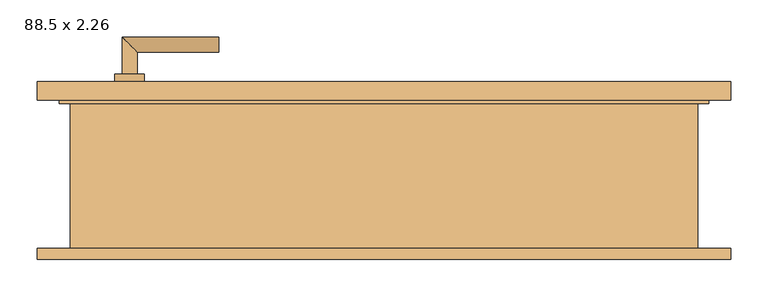
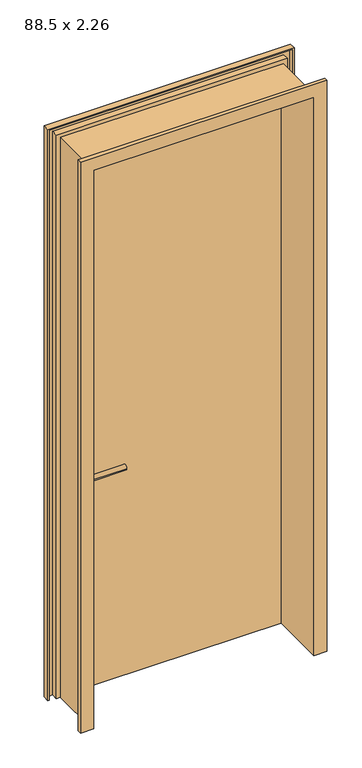
"""IFC4 building model written with IfcOpenShell, lengths in millimetres: door geometry, Drehflügel 1-flg - Stahlzarge : 88.5 x 2.26."""

from ifc_helpers import new_model, si_unit, point, frame, frame_2d, origin, origin_with_axes, place, context, project, spatial, polyline, circle_curve, ellipse_curve, trimmed, segment, composite_curve, outline, extrude, faceted_brep, source, transform, mapped, element, save
from ifc_brep_helpers import plane_surface, cylinder_surface, advanced_brep


def door_88_5_x_2_26_7d47f87c(model_context):
    return source(origin(), model_context, "Body", "SolidModel", [
        advanced_brep(
        [(-352.5, 89.4346141, 900.0), (-332.5, 89.4346141, 900.0), (-352.5, 19.4346141, 900.0), (-332.5, 39.4346141, 900.0), (-222.5, 19.4346141, 900.0), (-222.5, 39.4346141, 900.0)],
        [
            (0, 1, circle_curve(frame((-342.5, 89.4346141, 900.0), z_axis=(0.0, 1.0, 0.0), x_axis=(1.0, 0.0, 0.0)), 10.0)),
            (1, 0, circle_curve(frame((-342.5, 89.4346141, 900.0), z_axis=(0.0, 1.0, 0.0), x_axis=(1.0, 0.0, 0.0)), 10.0)),
            (0, 2),
            (2, 3, ellipse_curve(frame((-342.5, 29.4346141, 900.0), z_axis=(-0.7071067811865385, 0.7071067811865565, 0.0), x_axis=(0.7071067811865563, 0.7071067811865386, 0.0)), 14.1421356, 10.0)),
            (3, 1),
            (3, 2, ellipse_curve(frame((-342.5, 29.4346141, 900.0), z_axis=(-0.7071067811865385, 0.7071067811865565, 0.0), x_axis=(0.7071067811865563, 0.7071067811865386, 0.0)), 14.1421356, 10.0)),
            (4, 5, circle_curve(frame((-222.5, 29.4346141, 900.0), z_axis=(1.0, 0.0, 0.0), x_axis=(0.0, 1.0, 0.0)), 10.0)),
            (5, 4, circle_curve(frame((-222.5, 29.4346141, 900.0), z_axis=(1.0, 0.0, 0.0), x_axis=(0.0, 1.0, 0.0)), 10.0)),
            (2, 4),
            (5, 3),
        ],
        [
            plane_surface(frame((-342.5, 89.4346141, -387.7526403), z_axis=(0.0, 1.0, 0.0), x_axis=(0.0, 0.0, 1.0))),
            cylinder_surface(frame((-342.5, 89.4346141, 900.0), z_axis=(0.0, 1.0, 0.0), x_axis=(1.0, 0.0, 0.0)), 10.0),
            plane_surface(frame((-222.5, 29.4346141, -387.7526403), z_axis=(1.0, 0.0, 0.0), x_axis=(0.0, 0.0, 1.0))),
            cylinder_surface(frame((-342.5, 29.4346141, 900.0), z_axis=(-1.0, 0.0, 0.0), x_axis=(0.0, 1.0, 0.0)), 10.0),
        ],
        [
            (0, [[1, 2]]),
            (1, [[-1, 3, 4, 5]]),
            (1, [[-2, -5, 6, -3]]),
            (2, [[7, 8]]),
            (3, [[-4, 9, -8, 10]]),
            (3, [[-6, -10, -7, -9]]),
        ],
    ),
        advanced_brep(
        [(-332.5, 149.4346141, 900.0), (-352.5, 149.4346141, 900.0), (-332.5, 179.4346141, 900.0), (-352.5, 199.4346141, 900.0), (-222.5, 179.4346141, 900.0), (-222.5, 199.4346141, 900.0)],
        [
            (0, 1, circle_curve(frame((-342.5, 149.4346141, 900.0), z_axis=(0.0, -1.0, 0.0), x_axis=(-1.0, 0.0, 0.0)), 10.0)),
            (1, 0, circle_curve(frame((-342.5, 149.4346141, 900.0), z_axis=(0.0, -1.0, 0.0), x_axis=(-1.0, 0.0, 0.0)), 10.0)),
            (0, 2),
            (2, 3, ellipse_curve(frame((-342.5, 189.4346141, 900.0), z_axis=(-0.7071067811865475, -0.7071067811865475, 0.0), x_axis=(0.7071067811865474, -0.7071067811865476, 0.0)), 14.1421356, 10.0)),
            (3, 1),
            (3, 2, ellipse_curve(frame((-342.5, 189.4346141, 900.0), z_axis=(-0.7071067811865475, -0.7071067811865475, 0.0), x_axis=(0.7071067811865474, -0.7071067811865476, 0.0)), 14.1421356, 10.0)),
            (4, 5, circle_curve(frame((-222.5, 189.4346141, 900.0), z_axis=(1.0, 0.0, 0.0), x_axis=(0.0, 1.0, 0.0)), 10.0)),
            (5, 4, circle_curve(frame((-222.5, 189.4346141, 900.0), z_axis=(1.0, 0.0, 0.0), x_axis=(0.0, 1.0, 0.0)), 10.0)),
            (2, 4),
            (5, 3),
        ],
        [
            plane_surface(frame((-342.5, 149.4346141, -387.7526403), z_axis=(0.0, -1.0, 0.0), x_axis=(0.0, 0.0, 1.0))),
            cylinder_surface(frame((-342.5, 149.4346141, 900.0), z_axis=(0.0, -1.0, 0.0), x_axis=(-1.0, 0.0, 0.0)), 10.0),
            plane_surface(frame((-222.5, 189.4346141, -387.7526403), z_axis=(1.0, 0.0, 0.0), x_axis=(0.0, 0.0, 1.0))),
            cylinder_surface(frame((-342.5, 189.4346141, 900.0), z_axis=(-1.0, 0.0, 0.0), x_axis=(0.0, 1.0, 0.0)), 10.0),
        ],
        [
            (0, [[1, 2]]),
            (1, [[-1, 3, 4, 5]]),
            (1, [[-2, -5, 6, -3]]),
            (2, [[7, 8]]),
            (3, [[-4, 9, -8, 10]]),
            (3, [[-6, -10, -7, -9]]),
        ],
    ),
        extrude(outline(composite_curve([segment(trimmed(circle_curve(frame_2d((900.0, -342.5)), 20.0), [point((900.0, -362.5))], [point((900.0, -322.5))], False, "CARTESIAN"), True, "CONTINUOUS"), segment(trimmed(circle_curve(frame_2d((900.0, -342.5)), 20.0), [point((900.0, -322.5))], [point((900.0, -362.5))], False, "CARTESIAN"), True, "CONTINUOUS")], self_intersect=False)), frame((0.0, 79.4346141, 0.0), z_axis=(0.0, 1.0, 0.0), x_axis=(0.0, 0.0, 1.0)), (0.0, 0.0, 1.0), 10.0),
        extrude(outline(composite_curve([segment(trimmed(circle_curve(frame_2d((900.0, -342.5)), 20.0), [point((900.0, -362.5))], [point((900.0, -322.5))], False, "CARTESIAN"), True, "CONTINUOUS"), segment(trimmed(circle_curve(frame_2d((900.0, -342.5)), 20.0), [point((900.0, -322.5))], [point((900.0, -362.5))], False, "CARTESIAN"), True, "CONTINUOUS")], self_intersect=False)), frame((0.0, 139.4346141, 0.0), z_axis=(0.0, 1.0, 0.0), x_axis=(0.0, 0.0, 1.0)), (0.0, 0.0, 1.0), 10.0),
        extrude(outline(polyline([(432.5, 114.4346141), (-432.5, 114.4346141), (-432.5, 139.4346141), (432.5, 139.4346141), (432.5, 114.4346141)])), origin_with_axes(), (0.0, 0.0, 1.0), 2250.0),
        faceted_brep([(466.9603207, -100.5653859, 0.0), (417.5, -100.5653859, 0.0), (417.5, 114.4346141, 0.0), (432.5, 114.4346141, 0.0), (432.5, 139.4346141, 0.0), (466.9603207, 139.4346141, 0.0), (466.9603207, 114.4346141, 0.0), (461.9603207, 114.4346141, 0.0), (461.9603207, 134.4346141, 0.0), (437.5, 134.4346141, 0.0), (437.5, 109.4346141, 0.0), (422.5, 109.4346141, 0.0), (422.5, -95.5653859, 0.0), (461.9603207, -95.5653859, 0.0), (461.9603207, -85.5653859, 0.0), (466.9603207, -85.5653859, 0.0), (466.9603207, -100.5653859, 2284.4603207), (-466.9603207, -100.5653859, 2284.4603207), (-466.9603207, -100.5653859, 0.0), (-417.5, -100.5653859, 0.0), (-417.5, -100.5653859, 2235.0), (417.5, -100.5653859, 2235.0), (417.5, 114.4346141, 2235.0), (-417.5, 114.4346141, 2235.0), (-417.5, 114.4346141, 0.0), (-432.5, 114.4346141, 0.0), (-432.5, 114.4346141, 2250.0), (432.5, 114.4346141, 2250.0), (432.5, 139.4346141, 2250.0), (-432.5, 139.4346141, 2250.0), (-432.5, 139.4346141, 0.0), (-466.9603207, 139.4346141, 0.0), (-466.9603207, 139.4346141, 2284.4603207), (466.9603207, 139.4346141, 2284.4603207), (466.9603207, 114.4346141, 2284.4603207), (-466.9603207, 114.4346141, 2284.4603207), (-466.9603207, 114.4346141, 0.0), (-461.9603207, 114.4346141, 0.0), (-461.9603207, 114.4346141, 2279.4603207), (461.9603207, 114.4346141, 2279.4603207), (461.9603207, 134.4346141, 2279.4603207), (-461.9603207, 134.4346141, 2279.4603207), (-461.9603207, 134.4346141, 0.0), (-437.5, 134.4346141, 0.0), (-437.5, 134.4346141, 2255.0), (437.5, 134.4346141, 2255.0), (437.5, 109.4346141, 2255.0), (-437.5, 109.4346141, 2255.0), (-437.5, 109.4346141, 0.0), (-422.5, 109.4346141, 0.0), (-422.5, 109.4346141, 2240.0), (422.5, 109.4346141, 2240.0), (422.5, -95.5653859, 2240.0), (-422.5, -95.5653859, 2240.0), (-422.5, -95.5653859, 0.0), (-461.9603207, -95.5653859, 0.0), (-461.9603207, -95.5653859, 2279.4603207), (461.9603207, -95.5653859, 2279.4603207), (461.9603207, -85.5653859, 2279.4603207), (-461.9603207, -85.5653859, 2279.4603207), (-461.9603207, -85.5653859, 0.0), (-466.9603207, -85.5653859, 0.0), (-466.9603207, -85.5653859, 2284.4603207), (466.9603207, -85.5653859, 2284.4603207)], [[[0, 1, 2, 3, 4, 5, 6, 7, 8, 9, 10, 11, 12, 13, 14, 15]], [[1, 0, 16, 17, 18, 19, 20, 21]], [[2, 1, 21, 22]], [[3, 2, 22, 23, 24, 25, 26, 27]], [[4, 3, 27, 28]], [[5, 4, 28, 29, 30, 31, 32, 33]], [[6, 5, 33, 34]], [[7, 6, 34, 35, 36, 37, 38, 39]], [[8, 7, 39, 40]], [[9, 8, 40, 41, 42, 43, 44, 45]], [[10, 9, 45, 46]], [[11, 10, 46, 47, 48, 49, 50, 51]], [[12, 11, 51, 52]], [[13, 12, 52, 53, 54, 55, 56, 57]], [[14, 13, 57, 58]], [[15, 14, 58, 59, 60, 61, 62, 63]], [[0, 15, 63, 16]], [[17, 62, 61, 18]], [[18, 61, 60, 55, 54, 49, 48, 43, 42, 37, 36, 31, 30, 25, 24, 19]], [[23, 20, 19, 24]], [[29, 26, 25, 30]], [[35, 32, 31, 36]], [[41, 38, 37, 42]], [[47, 44, 43, 48]], [[53, 50, 49, 54]], [[59, 56, 55, 60]], [[22, 21, 20, 23]], [[28, 27, 26, 29]], [[34, 33, 32, 35]], [[40, 39, 38, 41]], [[46, 45, 44, 47]], [[52, 51, 50, 53]], [[58, 57, 56, 59]], [[16, 63, 62, 17]]]),
    ])


if __name__ == "__main__":
    model = new_model("IFC4")
    model_context = context("Model", 3, world=origin())
    ifc_project = project(units=[si_unit("LENGTHUNIT", "METRE", prefix="MILLI")], contexts=[model_context])
    site = spatial("IfcSite", under=ifc_project)
    building = spatial("IfcBuilding", under=site)
    placement = place(None, origin())
    door_88_5_x_2_26_shape = door_88_5_x_2_26_7d47f87c(model_context)
    element("IfcDoor", 1, ObjectType="Drehflügel 1-flg - Stahlzarge : 88.5 x 2.26", at=placement, inside=building, context=model_context, shape_type="MappedRepresentation", body=[
        mapped(door_88_5_x_2_26_shape, transform((0.0, 0.0, 0.0), x_axis=(1.0, 0.0, 0.0), y_axis=(0.0, 1.0, 0.0), z_axis=(0.0, 0.0, 1.0))),
    ])
    save(model, "model.ifc")

# Revit data of these elements
# Type "Drehflügel 1-flg - Stahlzarge : 88.5 x 2.26"
#   Construction Type Id = "opn-d38"
#   Type Mark = "20"
#   Operation = "SingleSwingRight"
#   Keynote = "16.03"
#   Analytic Construction = "Türfüllung Holz, Sturmtür Metall"
#   Thermal Resistance (R) = 0.270117 (m²·K)/W
#   Heat Transfer Coefficient (U) = 2.3279 W/(m²·K)
#   Rough Width = 0.885 m
#   Rough Height [instance default] = 2.360 m
#   Höhe Türgriff [instance default] = 0.900 m
#   Height = 2.260 m
#   Fußbodenaufbau [instance default] = 0.100 m
#   Width = 0.885 m
#   Sichtbarkeit Sturzlinien [instance default] = yes
#   Türgriff auswählen [instance default] = element 221079
#   Türgriff [instance default] = none
#   Türflügel [instance default] = none
#   Rahmen/Pfosten [instance default] = Metall - Lackiert - Grau
#   Visual Light Transmittance = 0
#   Solar Heat Gain Coefficient = 0
#   Function = (empty or 0)
#   Wall Closure = (empty or 0)
# Element 1 (IfcDoor, "Drehflügel 1-flg - Stahlzarge : 88.5 x 2.26")
#   Rough Height = 2.260 m
#   Fußbodenaufbau = 0.000 m
#   Materials on its faces: "Metall - Lackiert - Grau", "Metall - Chrom", "Holz - Birke"
# Materials
#   "Metall - Lackiert - Grau": class "Farbe 1", colour RGB 98 98 98, transparency 0, Cost = 0
#   "Metall - Chrom": class "Metall", colour RGB 247 247 247, transparency 0, Cost = 0
#   "Holz - Birke": class "Holz", colour RGB 213 164 103, transparency 0, Cost = 0
